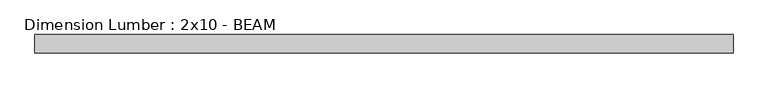
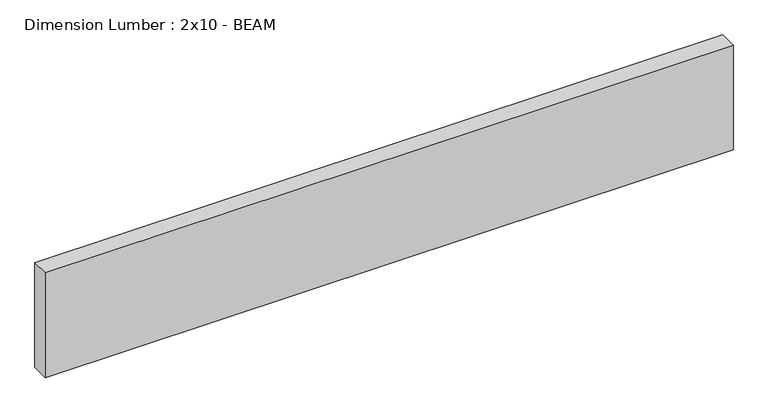
"""IFC4 building model written with IfcOpenShell, lengths in millimetres: beam geometry, Dimension Lumber : 2x10 - BEAM."""

from ifc_helpers import new_model, si_unit, frame, origin, place, context, project, spatial, polyline, outline, extrude, source, transform, mapped, element, save


def dimension_lumber_2x10_beam_fc7aac63(model_context):
    return source(origin(), model_context, "Body", "SweptSolid", [
        extrude(outline(polyline([(730.25, 19.05), (730.25, -19.05), (-730.25, -19.05), (-730.25, 19.05), (730.25, 19.05)])), frame((0.0, 0.0, -117.475), z_axis=(0.0, 0.0, 1.0), x_axis=(1.0, 0.0, 0.0)), (0.0, 0.0, 1.0), 234.95),
    ])


if __name__ == "__main__":
    model = new_model("IFC4")
    model_context = context("Model", 3, world=origin())
    ifc_project = project(units=[si_unit("LENGTHUNIT", "METRE", prefix="MILLI")], contexts=[model_context])
    site = spatial("IfcSite", under=ifc_project)
    building = spatial("IfcBuilding", under=site)
    placement = place(None, origin())
    dimension_lumber_2x10_beam_shape = dimension_lumber_2x10_beam_fc7aac63(model_context)
    element("IfcBeam", 1, ObjectType="Dimension Lumber : 2x10 - BEAM", at=placement, inside=building, context=model_context, shape_type="MappedRepresentation", body=[
        mapped(dimension_lumber_2x10_beam_shape, transform((0.0, 0.0, 0.0), x_axis=(1.0, 0.0, 0.0), y_axis=(0.0, 1.0, 0.0), z_axis=(0.0, 0.0, 1.0))),
    ])
    save(model, "model.ifc")

# Revit data of these elements
# Type "Dimension Lumber : 2x10 - BEAM"
#   Assembly Code = "B10"
#   A = 0.0755556 SF
#   Length [instance default] = 5' - 0"
#   b = 0' - 1 1/2"
#   d = 0' - 9 1/4"
#   Structural Material = (3) SISTERED 2X10s AT BEAM
# Element 1 (IfcBeam, "Dimension Lumber : 2x10 - BEAM")
#   Materials on its faces: "(3) SISTERED 2X10s AT BEAM"
# Materials
#   "(3) SISTERED 2X10s AT BEAM": class "Wood", colour RGB 234 198 147, transparency 0, Description = "Pinus Echinata", Cost = 0
